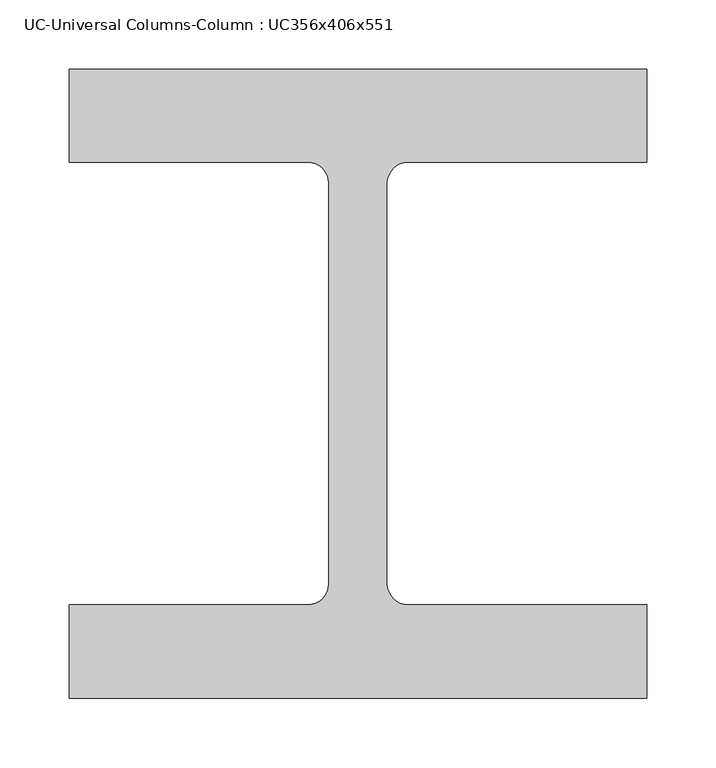
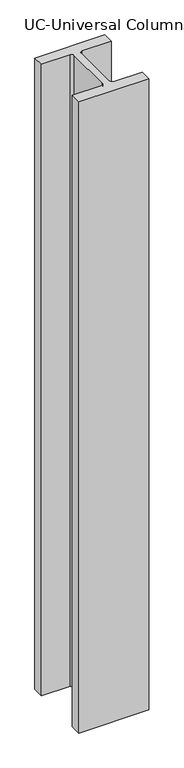
"""IFC4 building model written with IfcOpenShell, lengths in millimetres: column geometry, UC-Universal Columns-Column : UC356x406x551."""

import ifcopenshell
import ifcopenshell.guid

model = None  # the IFC model being written
_history = None  # IfcOwnerHistory: only IFC2X3 demands one
_inside = {}  # id of a spatial element -> (the spatial element, [elements in it])
_under = {}  # id of a project, library or spatial element -> (it, [spatial elements below it])
_declared = {}  # id of a project -> (the project, [libraries it declares])
_typed = {}  # id of a type object -> (the type object, [elements of that type])
_made_of = {}  # id of a material, layer set ... -> (it, [elements and type objects made of it])


def new_model(schema):
    """Start an empty IFC model of exactly this schema.

    Asked for "IFC4X3", IfcOpenShell would pick the latest addendum, in which some entities
    have other attributes; the version numbers below select the first issue.
    IFC2X3 requires an IfcOwnerHistory on every rooted entity: one is made here for all.
    """
    global model, _history
    if schema == "IFC4X3":
        model = ifcopenshell.file(schema_version=(4, 3, 0, 0))
    else:
        model = ifcopenshell.file(schema=schema)
    _inside.clear()
    _under.clear()
    _declared.clear()
    _typed.clear()
    _made_of.clear()
    _history = None
    if model.schema == "IFC2X3":
        org = make("IfcOrganization", Name="unknown")
        user = make(
            "IfcPersonAndOrganization",
            ThePerson=make("IfcPerson", FamilyName="unknown"),
            TheOrganization=org,
        )
        app = make(
            "IfcApplication",
            ApplicationDeveloper=org,
            Version="unknown",
            ApplicationFullName="unknown",
            ApplicationIdentifier="unknown",
        )
        _history = make(
            "IfcOwnerHistory",
            OwningUser=user,
            OwningApplication=app,
            ChangeAction="ADDED",
            CreationDate=0,
        )
    return model


def make(cls, **values):
    """One entity of the class cls with the attributes given. An attribute that is None is left unset."""
    return model.create_entity(
        cls, **{name: value for name, value in values.items() if value is not None}
    )


def rooted(cls, **values):
    """An entity with a GlobalId (a new one), such as an element, a storey or a relation."""
    return make(cls, GlobalId=ifcopenshell.guid.new(), OwnerHistory=_history, **values)


def si_unit(unit_type, name, prefix=None):
    """IfcSIUnit, for example si_unit("LENGTHUNIT", "METRE", prefix="MILLI")."""
    return make("IfcSIUnit", UnitType=unit_type, Prefix=prefix, Name=name)


def assignment(units):
    """IfcUnitAssignment: the units of a project."""
    return None if units is None else make("IfcUnitAssignment", Units=units)


def point(xyz):
    """IfcCartesianPoint."""
    return None if xyz is None else make("IfcCartesianPoint", Coordinates=xyz)


def direction(xyz):
    """IfcDirection."""
    return None if xyz is None else make("IfcDirection", DirectionRatios=xyz)


def frame(location, z_axis=None, x_axis=None):
    """IfcAxis2Placement3D, a coordinate frame: its origin and axes. An axis left out is left unset."""
    return make(
        "IfcAxis2Placement3D",
        Location=point(location),
        Axis=direction(z_axis),
        RefDirection=direction(x_axis),
    )


def frame_2d(location, x_axis=None):
    """IfcAxis2Placement2D, a coordinate frame in the plane: its origin and x axis."""
    return make(
        "IfcAxis2Placement2D", Location=point(location), RefDirection=direction(x_axis)
    )


def origin():
    """The frame at (0, 0, 0) with its axes left unset."""
    return frame((0.0, 0.0, 0.0))


def origin_with_axes():
    """The frame at (0, 0, 0) with the z axis (0, 0, 1) and the x axis (1, 0, 0) written out."""
    return frame((0.0, 0.0, 0.0), z_axis=(0.0, 0.0, 1.0), x_axis=(1.0, 0.0, 0.0))


def place(relative_to, where):
    """IfcLocalPlacement: puts the frame where relative to a parent placement (None: the world)."""
    return make(
        "IfcLocalPlacement", PlacementRelTo=relative_to, RelativePlacement=where
    )


def context(
    kind, dimensions, precision=None, world=None, true_north=None, identifier=None
):
    """IfcGeometricRepresentationContext, for example the 3D "Model" context."""
    return make(
        "IfcGeometricRepresentationContext",
        ContextIdentifier=identifier,
        ContextType=kind,
        CoordinateSpaceDimension=dimensions,
        Precision=precision,
        WorldCoordinateSystem=world,
        TrueNorth=true_north,
    )


def project(units=None, contexts=None):
    """IfcProject with its units and contexts."""
    return rooted(
        "IfcProject",
        Name="project",
        RepresentationContexts=contexts,
        UnitsInContext=assignment(units),
    )


def spatial(cls, under=None, at=None, **own):
    """A site, building, storey or space (cls), placed at a placement, below another one or the project."""
    s = rooted(cls, ObjectPlacement=at, **own)
    if under is not None:
        _under.setdefault(under.id(), (under, []))[1].append(s)
    return s


def polyline(points):
    """IfcPolyline through the points."""
    return make("IfcPolyline", Points=[point(p) for p in points])


def circle_curve(where, radius):
    """IfcCircle in the frame where."""
    return make("IfcCircle", Position=where, Radius=radius)


def trimmed(basis, trim1, trim2, sense, master):
    """IfcTrimmedCurve: the piece of a basis curve between two trims."""
    return make(
        "IfcTrimmedCurve",
        BasisCurve=basis,
        Trim1=trim1,
        Trim2=trim2,
        SenseAgreement=sense,
        MasterRepresentation=master,
    )


def segment(curve, same_sense, transition):
    """IfcCompositeCurveSegment."""
    return make(
        "IfcCompositeCurveSegment",
        Transition=transition,
        SameSense=same_sense,
        ParentCurve=curve,
    )


def composite_curve(segments, self_intersect=None):
    """IfcCompositeCurve: segments joined end to end."""
    return make("IfcCompositeCurve", Segments=segments, SelfIntersect=self_intersect)


def outline(outer, holes=None, kind="AREA"):
    """IfcArbitraryClosedProfileDef: a profile drawn as a closed curve; with holes, ...WithVoids."""
    if holes is None:
        return make("IfcArbitraryClosedProfileDef", ProfileType=kind, OuterCurve=outer)
    return make(
        "IfcArbitraryProfileDefWithVoids",
        ProfileType=kind,
        OuterCurve=outer,
        InnerCurves=holes,
    )


def extrude(swept, where, along, depth):
    """IfcExtrudedAreaSolid: the profile swept, set in the frame where, extruded along a direction by depth."""
    return make(
        "IfcExtrudedAreaSolid",
        SweptArea=swept,
        Position=where,
        ExtrudedDirection=direction(along),
        Depth=depth,
    )


def shape(context_of_items, identifier, shape_type, items):
    """IfcShapeRepresentation: the items that make up one representation, for example the "Body"."""
    return make(
        "IfcShapeRepresentation",
        ContextOfItems=context_of_items,
        RepresentationIdentifier=identifier,
        RepresentationType=shape_type,
        Items=items,
    )


def source(mapping_origin, context_of_items, identifier, shape_type, items):
    """IfcRepresentationMap: a shape defined once, which mapped items show again and again."""
    return make(
        "IfcRepresentationMap",
        MappingOrigin=mapping_origin,
        MappedRepresentation=shape(context_of_items, identifier, shape_type, items),
    )


def transform(
    local_origin,
    x_axis=None,
    y_axis=None,
    z_axis=None,
    scale=None,
    scale2=None,
    scale3=None,
    uniform=True,
):
    """IfcCartesianTransformationOperator3D, or its non-uniform kind. x_axis, y_axis, z_axis: its Axis1, 2, 3."""
    if uniform:
        return make(
            "IfcCartesianTransformationOperator3D",
            Axis1=direction(x_axis),
            Axis2=direction(y_axis),
            LocalOrigin=point(local_origin),
            Scale=scale,
            Axis3=direction(z_axis),
        )
    return make(
        "IfcCartesianTransformationOperator3DnonUniform",
        Axis1=direction(x_axis),
        Axis2=direction(y_axis),
        LocalOrigin=point(local_origin),
        Scale=scale,
        Axis3=direction(z_axis),
        Scale2=scale2,
        Scale3=scale3,
    )


def mapped(mapping_source, mapping_target):
    """IfcMappedItem: shows the shape of a source again, moved by a transform."""
    return make(
        "IfcMappedItem", MappingSource=mapping_source, MappingTarget=mapping_target
    )


def made_of(thing, what):
    """Note that an element or type object is made of a material, layer set ...; save() writes the relation."""
    if what is not None:
        _made_of.setdefault(what.id(), (what, []))[1].append(thing)
    return thing


def element(
    cls,
    number,
    at=None,
    inside=None,
    cuts=None,
    type_object=None,
    material=None,
    context=None,
    identifier="Body",
    shape_type=None,
    held_by="IfcProductDefinitionShape",
    body=None,
    shapes=None,
    **own,
):
    """One element of the class cls, such as IfcWall. Its Tag is "e" and its number.

    at: its placement. inside: the storey or other place that contains it. cuts: it is an
    opening in that element (IfcRelVoidsElement). A single representation is given by context,
    identifier, shape_type and body (its items); several are given by shapes. held_by: the class
    of the entity that holds the representations. save() writes the other relations.
    """
    e = rooted(cls, Tag="e%d" % number, ObjectPlacement=at, **own)
    if body is not None:
        shapes = [shape(context, identifier, shape_type, body)]
    if shapes is not None:
        e.Representation = make(held_by, Representations=shapes)
    if inside is not None:
        _inside.setdefault(inside.id(), (inside, []))[1].append(e)
    if cuts is not None:
        rooted(
            "IfcRelVoidsElement", RelatingBuildingElement=cuts, RelatedOpeningElement=e
        )
    if type_object is not None:
        _typed.setdefault(type_object.id(), (type_object, []))[1].append(e)
    return made_of(e, material)


def aggregate(whole, parts):
    """IfcRelAggregates: a whole, such as a stair, and the parts it consists of."""
    return rooted("IfcRelAggregates", RelatingObject=whole, RelatedObjects=parts)


def save(model, path):
    """Write the relations noted so far, then the file.

    IfcRelAggregates (storeys below a building ...), IfcRelContainedInSpatialStructure (elements
    in a storey), IfcRelDefinesByType, IfcRelAssociatesMaterial and IfcRelDeclares: one each for
    every whole, place, type object, material and project.
    """
    for whole, parts in _under.values():
        aggregate(whole, parts)
    for where, things in _inside.values():
        rooted(
            "IfcRelContainedInSpatialStructure",
            RelatedElements=things,
            RelatingStructure=where,
        )
    for kind, things in _typed.values():
        rooted("IfcRelDefinesByType", RelatedObjects=things, RelatingType=kind)
    for what, things in _made_of.values():
        rooted("IfcRelAssociatesMaterial", RelatedObjects=things, RelatingMaterial=what)
    for by, libraries in _declared.values():
        rooted("IfcRelDeclares", RelatingContext=by, RelatedDefinitions=libraries)
    model.write(path)


def uc_universal_columns_column_uc356x406x551_b8cfbe81(model_context):
    return source(origin(), model_context, "Body", "SweptSolid", [
        extrude(outline(composite_curve([segment(polyline([(209.25, 227.8), (209.25, 160.3), (36.25, 160.3)]), True, "CONTINUOUS"), segment(trimmed(circle_curve(frame_2d((36.25, 145.1)), 15.2), [point((36.25, 160.3))], [point((21.05, 145.1))], True, "CARTESIAN"), True, "CONTINUOUS"), segment(polyline([(21.05, 145.1), (21.05, -145.1)]), True, "CONTINUOUS"), segment(trimmed(circle_curve(frame_2d((36.25, -145.1)), 15.2), [point((21.05, -145.1))], [point((36.25, -160.3))], True, "CARTESIAN"), True, "CONTINUOUS"), segment(polyline([(36.25, -160.3), (209.25, -160.3), (209.25, -227.8), (-209.25, -227.8), (-209.25, -160.3), (-36.25, -160.3)]), True, "CONTINUOUS"), segment(trimmed(circle_curve(frame_2d((-36.25, -145.1)), 15.2), [point((-36.25, -160.3))], [point((-21.05, -145.1))], True, "CARTESIAN"), True, "CONTINUOUS"), segment(polyline([(-21.05, -145.1), (-21.05, 145.1)]), True, "CONTINUOUS"), segment(trimmed(circle_curve(frame_2d((-36.25, 145.1)), 15.2), [point((-21.05, 145.1))], [point((-36.25, 160.3))], True, "CARTESIAN"), True, "CONTINUOUS"), segment(polyline([(-36.25, 160.3), (-209.25, 160.3), (-209.25, 227.8), (209.25, 227.8)]), True, "CONTINUOUS")], self_intersect=False)), origin_with_axes(), (0.0, 0.0, 1.0), 4000.0),
    ])


if __name__ == "__main__":
    model = new_model("IFC4")
    model_context = context("Model", 3, world=origin())
    ifc_project = project(units=[si_unit("LENGTHUNIT", "METRE", prefix="MILLI")], contexts=[model_context])
    site = spatial("IfcSite", under=ifc_project)
    building = spatial("IfcBuilding", under=site)
    placement = place(None, origin())
    uc_universal_columns_column_uc356x406x551_shape = uc_universal_columns_column_uc356x406x551_b8cfbe81(model_context)
    element("IfcColumn", 1, ObjectType="UC-Universal Columns-Column : UC356x406x551", at=placement, inside=building, context=model_context, shape_type="MappedRepresentation", body=[
        mapped(uc_universal_columns_column_uc356x406x551_shape, transform((0.0, 0.0, 0.0), x_axis=(1.0, 0.0, 0.0), y_axis=(0.0, 1.0, 0.0), z_axis=(0.0, 0.0, 1.0))),
    ])
    save(model, "model.ifc")

# Revit data of these elements
# Type "UC-Universal Columns-Column : UC356x406x551"
#   Section Name Key = "UC356x406x551"
#   Width = 41.85 cm
#   Web Thickness = 4.21 cm
#   Web Fillet = 1.52 cm
#   Warping Constant = 31100000.0 cm⁶
#   Torsional Moment of Inertia = 9240.00 cm⁴
#   Section Area = 702.0 cm²
#   Plastic Modulus weak axis = 6058.0 cm³
#   Plastic Modulus strong axis = 12076.0 cm³
#   Nominal Weight = 551.00 kgf/m
#   Moment of Inertia weak axis = 82671.00 cm⁴
#   Moment of Inertia strong axis = 226938.00 cm⁴
#   Height = 45.56 cm
#   Flange Thickness = 6.75 cm
#   Elastic Modulus weak axis = 3951.0 cm³
#   Elastic Modulus strong axis = 9962.0 cm³
#   Centroid Vertical = 22.78 cm
#   Centroid Horizontal = 20.925 cm
#   built-in parameter 1005541 = 0.246063 (stored number, unit not read)
#   built-in parameter 1005540 = 0.459318 (stored number, unit not read)
#   Bolt Spacing = 14.0 cm
#   Structural Material [instance default] = Metal - Steel 43-275
#   Type Comments = ""
#   Assembly Code = ""
# Element 1 (IfcColumn, "UC-Universal Columns-Column : UC356x406x551")
#   Materials on its faces: "Metal - Steel 43-275"
# Materials
#   "Metal - Steel 43-275": class "Metal", colour RGB 247 247 247, transparency 0, Cost = 0
